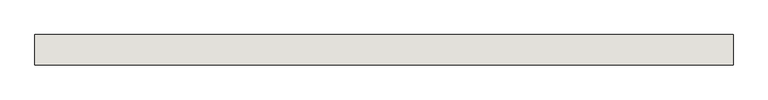
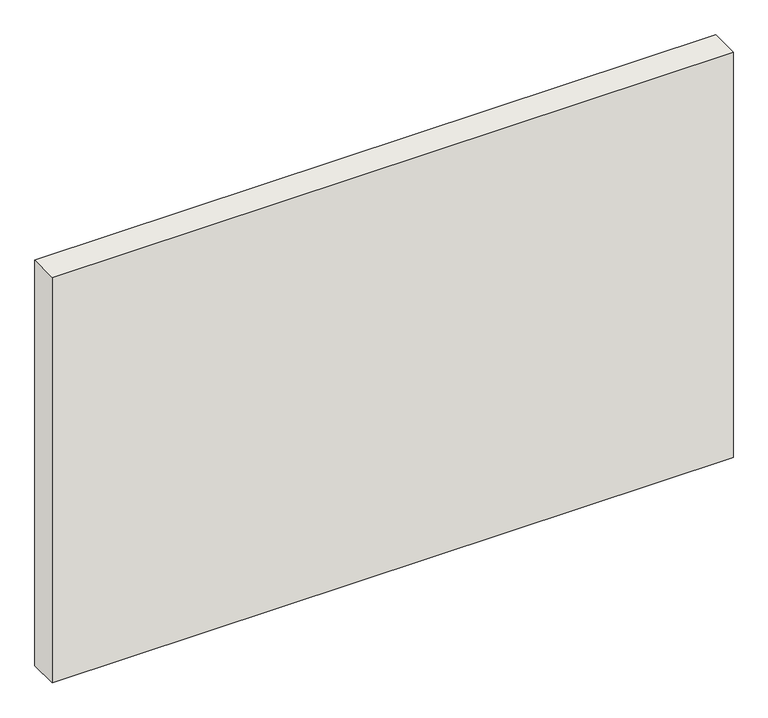
"""IFC4 building model written with IfcOpenShell, lengths in millimetres: wall geometry, Holzwand."""

from ifc_helpers import new_model, si_unit, origin, origin_with_axes, place, context, project, spatial, polyline, outline, extrude, source, transform, mapped, element, save


def wall_ab76accb(model_context):
    return source(origin(), model_context, "Body", "SweptSolid", [
        extrude(outline(polyline([(4570.0, 200.0), (4570.0, 0.0), (0.0, 0.0), (0.0, 200.0), (4570.0, 200.0)])), origin_with_axes(), (0.0, 0.0, 1.0), 2880.0),
    ])


if __name__ == "__main__":
    model = new_model("IFC4")
    model_context = context("Model", 3, world=origin())
    ifc_project = project(units=[si_unit("LENGTHUNIT", "METRE", prefix="MILLI")], contexts=[model_context])
    site = spatial("IfcSite", under=ifc_project)
    building = spatial("IfcBuilding", under=site)
    placement = place(None, origin())
    wall_shape = wall_ab76accb(model_context)
    element("IfcWall", 1, ObjectType="Holzwand", at=placement, inside=building, context=model_context, shape_type="MappedRepresentation", body=[
        mapped(wall_shape, transform((0.0, 0.0, 0.0), x_axis=(1.0, 0.0, 0.0), y_axis=(0.0, 1.0, 0.0), z_axis=(0.0, 0.0, 1.0))),
    ])
    save(model, "model.ifc")

# Revit data of these elements
# Element 1 (IfcWall, "Holzwand")
#   Materials on its faces: "holzschalung"
# Materials
#   "holzschalung": class "Unassigned", colour RGB 128 128 128, transparency 0
